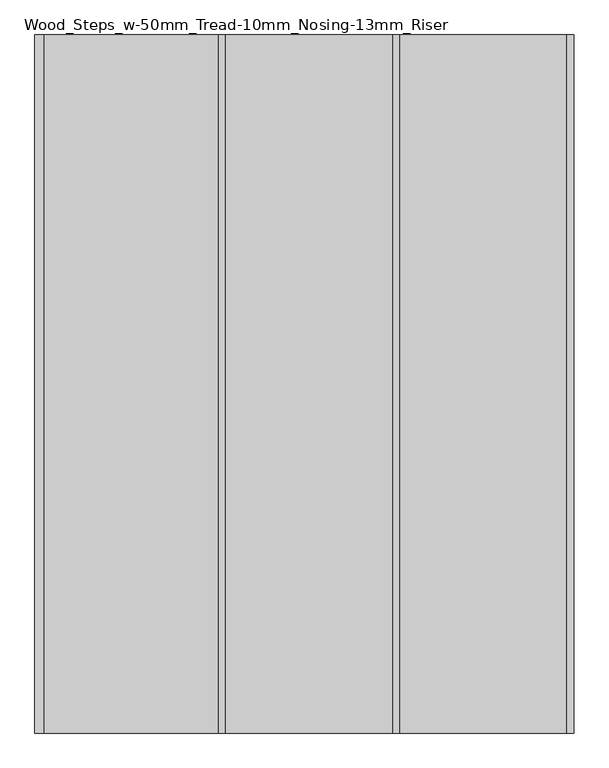
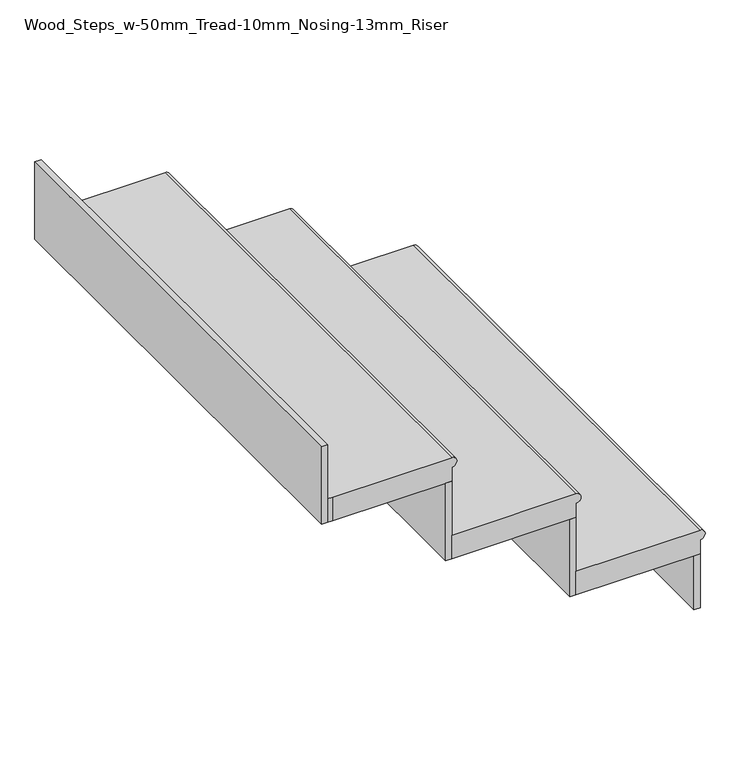
"""IFC4 building model written with IfcOpenShell, lengths in millimetres: stair flight geometry, Wood_Steps_w-50mm_Tread-10mm_Nosing-13mm_Riser."""

from ifc_helpers import new_model, si_unit, frame, origin, place, context, project, spatial, circle_curve, faceted_brep, source, transform, mapped, element, save
from ifc_brep_helpers import plane_surface, cylinder_surface, advanced_brep


def wood_steps_w_50mm_tread_10mm_nosing_13mm_riser_08b18785(model_context):
    return source(origin(), model_context, "Body", "SolidModel", [
        advanced_brep(
        [(-1845.8194784, -2645.3813072, 144.7058824), (-1845.8194784, -2645.3813072, 164.7058824), (-1845.8194784, -3645.3813072, 164.7058824), (-1845.8194784, -3645.3813072, 144.7058824), (-2095.8194784, -3645.3813072, 164.7058824), (-2095.8194784, -2645.3813072, 164.7058824), (-1845.8194784, -3645.3813072, 114.7058824), (-2095.8194784, -3645.3813072, 114.7058824), (-2095.8194784, -2645.3813072, 114.7058824), (-1845.8194784, -2645.3813072, 114.7058824)],
        [
            (0, 1, circle_curve(frame((-1845.8194784, -2645.3813072, 154.7058824), z_axis=(0.0, -1.0, 0.0), x_axis=(-1.0, 0.0, 0.0)), 10.0)),
            (1, 2),
            (2, 3, circle_curve(frame((-1845.8194784, -3645.3813072, 154.7058824), z_axis=(0.0, 1.0, 0.0), x_axis=(-1.0, 0.0, 0.0)), 10.0)),
            (3, 0),
            (4, 2),
            (1, 5),
            (5, 4),
            (6, 7),
            (7, 8),
            (8, 9),
            (9, 6),
            (4, 7),
            (6, 3),
            (9, 0),
            (8, 5),
        ],
        [
            cylinder_surface(frame((-1845.8194784, -2645.3813072, 154.7058824), z_axis=(0.0, 1.0, 0.0), x_axis=(-1.0, 0.0, 0.0)), 10.0),
            plane_surface(frame((-1835.8194784, -3645.3813072, 164.7058824), z_axis=(0.0, 0.0, 1.0), x_axis=(1.0, 0.0, 0.0))),
            plane_surface(frame((-1835.8194784, -3645.3813072, 114.7058824), z_axis=(0.0, 0.0, -1.0), x_axis=(-1.0, 0.0, 0.0))),
            plane_surface(frame((-2095.8194784, -3645.3813072, 164.7058824), z_axis=(0.0, -1.0, 0.0), x_axis=(0.0, 0.0, -1.0))),
            plane_surface(frame((-1845.8194784, -3645.3813072, 164.7058824), z_axis=(1.0, 0.0, 0.0), x_axis=(0.0, 0.0, -1.0))),
            plane_surface(frame((-1845.8194784, -2645.3813072, 164.7058824), z_axis=(0.0, 1.0, 0.0), x_axis=(0.0, 0.0, -1.0))),
            plane_surface(frame((-2095.8194784, -2645.3813072, 164.7058824), z_axis=(-1.0, 0.0, 0.0), x_axis=(0.0, 0.0, -1.0))),
        ],
        [
            (0, [[1, 2, 3, 4]]),
            (1, [[5, -2, 6, 7]]),
            (2, [[8, 9, 10, 11]]),
            (3, [[-5, 12, -8, 13, -3]]),
            (4, [[-11, 14, -4, -13]]),
            (5, [[-6, -1, -14, -10, 15]]),
            (6, [[-7, -15, -9, -12]]),
        ],
    ),
        faceted_brep([(-1845.8194784, -2645.3813072, 114.7058824), (-1845.8194784, -2645.3813072, 0.0), (-1858.3194784, -2645.3813072, 0.0), (-1858.3194784, -2645.3813072, 114.7058824), (-1845.8194784, -3645.3813072, 114.7058824), (-1858.3194784, -3645.3813072, 114.7058824), (-1858.3194784, -3645.3813072, 0.0), (-1845.8194784, -3645.3813072, 0.0)], [[[0, 1, 2, 3]], [[4, 5, 6, 7]], [[1, 0, 4, 7]], [[2, 1, 7, 6]], [[3, 2, 6, 5]], [[0, 3, 5, 4]]]),
        faceted_brep([(-2095.8194784, -2645.3813072, 279.4117647), (-2095.8194784, -2645.3813072, 114.7058824), (-2108.3194784, -2645.3813072, 114.7058824), (-2108.3194784, -2645.3813072, 279.4117647), (-2095.8194784, -3645.3813072, 279.4117647), (-2108.3194784, -3645.3813072, 279.4117647), (-2108.3194784, -3645.3813072, 114.7058824), (-2095.8194784, -3645.3813072, 114.7058824)], [[[0, 1, 2, 3]], [[4, 5, 6, 7]], [[1, 0, 4, 7]], [[2, 1, 7, 6]], [[3, 2, 6, 5]], [[0, 3, 5, 4]]]),
        advanced_brep(
        [(-2345.8194784, -3645.3813072, 329.4117647), (-2095.8194784, -3645.3813072, 329.4117647), (-2095.8194784, -2645.3813072, 329.4117647), (-2345.8194784, -2645.3813072, 329.4117647), (-2095.8194784, -3645.3813072, 279.4117647), (-2345.8194784, -3645.3813072, 279.4117647), (-2345.8194784, -2645.3813072, 279.4117647), (-2095.8194784, -2645.3813072, 279.4117647), (-2095.8194784, -3645.3813072, 309.4117647), (-2095.8194784, -2645.3813072, 309.4117647)],
        [
            (0, 1),
            (1, 2),
            (2, 3),
            (3, 0),
            (4, 5),
            (5, 6),
            (6, 7),
            (7, 4),
            (0, 5),
            (4, 8),
            (8, 1, circle_curve(frame((-2095.8194784, -3645.3813072, 319.4117647), z_axis=(0.0, -1.0, 0.0), x_axis=(-1.0, 0.0, 0.0)), 10.0)),
            (7, 9),
            (9, 8),
            (2, 9, circle_curve(frame((-2095.8194784, -2645.3813072, 319.4117647), z_axis=(0.0, 1.0, 0.0), x_axis=(-1.0, 0.0, 0.0)), 10.0)),
            (6, 3),
        ],
        [
            plane_surface(frame((-1835.8194784, -3645.3813072, 329.4117647), z_axis=(0.0, 0.0, 1.0), x_axis=(1.0, 0.0, 0.0))),
            plane_surface(frame((-1835.8194784, -3645.3813072, 279.4117647), z_axis=(0.0, 0.0, -1.0), x_axis=(-1.0, 0.0, 0.0))),
            plane_surface(frame((-2345.8194784, -3645.3813072, 329.4117647), z_axis=(0.0, -1.0, 0.0), x_axis=(0.0, 0.0, -1.0))),
            plane_surface(frame((-2095.8194784, -3645.3813072, 329.4117647), z_axis=(1.0, 0.0, 0.0), x_axis=(0.0, 0.0, -1.0))),
            plane_surface(frame((-2095.8194784, -2645.3813072, 329.4117647), z_axis=(0.0, 1.0, 0.0), x_axis=(0.0, 0.0, -1.0))),
            plane_surface(frame((-2345.8194784, -2645.3813072, 329.4117647), z_axis=(-1.0, 0.0, 0.0), x_axis=(0.0, 0.0, -1.0))),
            cylinder_surface(frame((-2095.8194784, -2645.3813072, 319.4117647), z_axis=(0.0, 1.0, 0.0), x_axis=(-1.0, 0.0, 0.0)), 10.0),
        ],
        [
            (0, [[1, 2, 3, 4]]),
            (1, [[5, 6, 7, 8]]),
            (2, [[-1, 9, -5, 10, 11]]),
            (3, [[-8, 12, 13, -10]]),
            (4, [[-3, 14, -12, -7, 15]]),
            (5, [[-4, -15, -6, -9]]),
            (6, [[-14, -2, -11, -13]]),
        ],
    ),
        faceted_brep([(-2595.8194784, -2645.3813072, 608.8235294), (-2595.8194784, -2645.3813072, 444.1176471), (-2608.3194784, -2645.3813072, 444.1176471), (-2608.3194784, -2645.3813072, 608.8235294), (-2595.8194784, -3645.3813072, 608.8235294), (-2608.3194784, -3645.3813072, 608.8235294), (-2608.3194784, -3645.3813072, 444.1176471), (-2595.8194784, -3645.3813072, 444.1176471)], [[[0, 1, 2, 3]], [[4, 5, 6, 7]], [[1, 0, 4, 7]], [[2, 1, 7, 6]], [[3, 2, 6, 5]], [[0, 3, 5, 4]]]),
        faceted_brep([(-2345.8194784, -2645.3813072, 444.1176471), (-2345.8194784, -2645.3813072, 279.4117647), (-2358.3194784, -2645.3813072, 279.4117647), (-2358.3194784, -2645.3813072, 444.1176471), (-2345.8194784, -3645.3813072, 444.1176471), (-2358.3194784, -3645.3813072, 444.1176471), (-2358.3194784, -3645.3813072, 279.4117647), (-2345.8194784, -3645.3813072, 279.4117647)], [[[0, 1, 2, 3]], [[4, 5, 6, 7]], [[1, 0, 4, 7]], [[2, 1, 7, 6]], [[3, 2, 6, 5]], [[0, 3, 5, 4]]]),
        advanced_brep(
        [(-2595.8194784, -3645.3813072, 494.1176471), (-2585.8194784, -3645.3813072, 494.1176471), (-2345.8194784, -3645.3813072, 494.1176471), (-2345.8194784, -2645.3813072, 494.1176471), (-2585.8194784, -2645.3813072, 494.1176471), (-2595.8194784, -2645.3813072, 494.1176471), (-2585.8194784, -3645.3813072, 444.1176471), (-2595.8194784, -3645.3813072, 444.1176471), (-2595.8194784, -2645.3813072, 444.1176471), (-2585.8194784, -2645.3813072, 444.1176471), (-2345.8194784, -2645.3813072, 444.1176471), (-2345.8194784, -3645.3813072, 444.1176471), (-2345.8194784, -3645.3813072, 474.1176471), (-2345.8194784, -2645.3813072, 474.1176471)],
        [
            (0, 1),
            (1, 2),
            (2, 3),
            (3, 4),
            (4, 5),
            (5, 0),
            (6, 7),
            (7, 8),
            (8, 9),
            (9, 10),
            (10, 11),
            (11, 6),
            (0, 7),
            (6, 1),
            (11, 12),
            (12, 2, circle_curve(frame((-2345.8194784, -3645.3813072, 484.1176471), z_axis=(0.0, -1.0, 0.0), x_axis=(-1.0, 0.0, 0.0)), 10.0)),
            (10, 13),
            (13, 12),
            (3, 13, circle_curve(frame((-2345.8194784, -2645.3813072, 484.1176471), z_axis=(0.0, 1.0, 0.0), x_axis=(-1.0, 0.0, 0.0)), 10.0)),
            (9, 4),
            (8, 5),
        ],
        [
            plane_surface(frame((-2585.8194784, -3645.3813072, 494.1176471), z_axis=(0.0, 0.0, 1.0), x_axis=(1.0, 0.0, 0.0))),
            plane_surface(frame((-2585.8194784, -3645.3813072, 444.1176471), z_axis=(0.0, 0.0, -1.0), x_axis=(-1.0, 0.0, 0.0))),
            plane_surface(frame((-2595.8194784, -3645.3813072, 494.1176471), z_axis=(0.0, -1.0, 0.0), x_axis=(0.0, 0.0, -1.0))),
            plane_surface(frame((-2585.8194784, -3645.3813072, 494.1176471), z_axis=(0.0, -1.0, 0.0), x_axis=(0.0, 0.0, -1.0))),
            plane_surface(frame((-2345.8194784, -3645.3813072, 494.1176471), z_axis=(1.0, 0.0, 0.0), x_axis=(0.0, 0.0, -1.0))),
            plane_surface(frame((-2345.8194784, -2645.3813072, 494.1176471), z_axis=(0.0, 1.0, 0.0), x_axis=(0.0, 0.0, -1.0))),
            plane_surface(frame((-2585.8194784, -2645.3813072, 494.1176471), z_axis=(0.0, 1.0, 0.0), x_axis=(0.0, 0.0, -1.0))),
            plane_surface(frame((-2595.8194784, -2645.3813072, 494.1176471), z_axis=(-1.0, 0.0, 0.0), x_axis=(0.0, 0.0, -1.0))),
            cylinder_surface(frame((-2345.8194784, -2645.3813072, 484.1176471), z_axis=(0.0, 1.0, 0.0), x_axis=(-1.0, 0.0, 0.0)), 10.0),
        ],
        [
            (0, [[1, 2, 3, 4, 5, 6]]),
            (1, [[7, 8, 9, 10, 11, 12]]),
            (2, [[-1, 13, -7, 14]]),
            (3, [[-2, -14, -12, 15, 16]]),
            (4, [[-11, 17, 18, -15]]),
            (5, [[-4, 19, -17, -10, 20]]),
            (6, [[-5, -20, -9, 21]]),
            (7, [[-6, -21, -8, -13]]),
            (8, [[-19, -3, -16, -18]]),
        ],
    ),
    ])


if __name__ == "__main__":
    model = new_model("IFC4")
    model_context = context("Model", 3, world=origin())
    ifc_project = project(units=[si_unit("LENGTHUNIT", "METRE", prefix="MILLI")], contexts=[model_context])
    site = spatial("IfcSite", under=ifc_project)
    building = spatial("IfcBuilding", under=site)
    placement = place(None, origin())
    wood_steps_w_50mm_tread_10mm_nosing_13mm_riser_shape = wood_steps_w_50mm_tread_10mm_nosing_13mm_riser_08b18785(model_context)
    element("IfcStairFlight", 1, ObjectType="Wood_Steps_w-50mm_Tread-10mm_Nosing-13mm_Riser", at=placement, inside=building, context=model_context, shape_type="MappedRepresentation", body=[
        mapped(wood_steps_w_50mm_tread_10mm_nosing_13mm_riser_shape, transform((0.0, 0.0, 0.0), x_axis=(1.0, 0.0, 0.0), y_axis=(0.0, 1.0, 0.0), z_axis=(0.0, 0.0, 1.0))),
    ])
    save(model, "model.ifc")

# Revit data of these elements
# Element 1 (IfcStairFlight, "Wood_Steps_w-50mm_Tread-10mm_Nosing-13mm_Riser")
#   Materials on its faces: "Oak Flooring"
# Materials
#   "Oak Flooring": class "Wood", colour RGB 212 179 113, transparency 0, Description = "Quercus Rubra", Cost = 0
